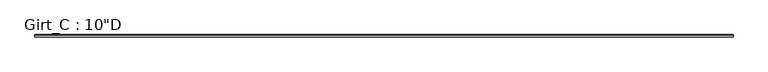
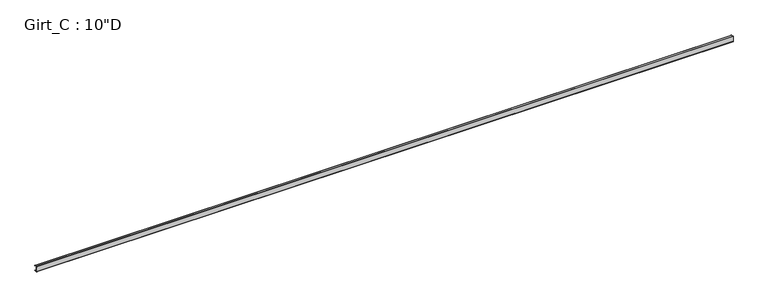
"""IFC4 building model written with IfcOpenShell, lengths in millimetres: beam geometry."""

import ifcopenshell
import ifcopenshell.guid

model = None  # the IFC model being written
_history = None  # IfcOwnerHistory: only IFC2X3 demands one
_inside = {}  # id of a spatial element -> (the spatial element, [elements in it])
_under = {}  # id of a project, library or spatial element -> (it, [spatial elements below it])
_declared = {}  # id of a project -> (the project, [libraries it declares])
_typed = {}  # id of a type object -> (the type object, [elements of that type])
_made_of = {}  # id of a material, layer set ... -> (it, [elements and type objects made of it])


def new_model(schema):
    """Start an empty IFC model of exactly this schema.

    Asked for "IFC4X3", IfcOpenShell would pick the latest addendum, in which some entities
    have other attributes; the version numbers below select the first issue.
    IFC2X3 requires an IfcOwnerHistory on every rooted entity: one is made here for all.
    """
    global model, _history
    if schema == "IFC4X3":
        model = ifcopenshell.file(schema_version=(4, 3, 0, 0))
    else:
        model = ifcopenshell.file(schema=schema)
    _inside.clear()
    _under.clear()
    _declared.clear()
    _typed.clear()
    _made_of.clear()
    _history = None
    if model.schema == "IFC2X3":
        org = make("IfcOrganization", Name="unknown")
        user = make(
            "IfcPersonAndOrganization",
            ThePerson=make("IfcPerson", FamilyName="unknown"),
            TheOrganization=org,
        )
        app = make(
            "IfcApplication",
            ApplicationDeveloper=org,
            Version="unknown",
            ApplicationFullName="unknown",
            ApplicationIdentifier="unknown",
        )
        _history = make(
            "IfcOwnerHistory",
            OwningUser=user,
            OwningApplication=app,
            ChangeAction="ADDED",
            CreationDate=0,
        )
    return model


def make(cls, **values):
    """One entity of the class cls with the attributes given. An attribute that is None is left unset."""
    return model.create_entity(
        cls, **{name: value for name, value in values.items() if value is not None}
    )


def rooted(cls, **values):
    """An entity with a GlobalId (a new one), such as an element, a storey or a relation."""
    return make(cls, GlobalId=ifcopenshell.guid.new(), OwnerHistory=_history, **values)


def si_unit(unit_type, name, prefix=None):
    """IfcSIUnit, for example si_unit("LENGTHUNIT", "METRE", prefix="MILLI")."""
    return make("IfcSIUnit", UnitType=unit_type, Prefix=prefix, Name=name)


def assignment(units):
    """IfcUnitAssignment: the units of a project."""
    return None if units is None else make("IfcUnitAssignment", Units=units)


def point(xyz):
    """IfcCartesianPoint."""
    return None if xyz is None else make("IfcCartesianPoint", Coordinates=xyz)


def direction(xyz):
    """IfcDirection."""
    return None if xyz is None else make("IfcDirection", DirectionRatios=xyz)


def frame(location, z_axis=None, x_axis=None):
    """IfcAxis2Placement3D, a coordinate frame: its origin and axes. An axis left out is left unset."""
    return make(
        "IfcAxis2Placement3D",
        Location=point(location),
        Axis=direction(z_axis),
        RefDirection=direction(x_axis),
    )


def frame_2d(location, x_axis=None):
    """IfcAxis2Placement2D, a coordinate frame in the plane: its origin and x axis."""
    return make(
        "IfcAxis2Placement2D", Location=point(location), RefDirection=direction(x_axis)
    )


def origin():
    """The frame at (0, 0, 0) with its axes left unset."""
    return frame((0.0, 0.0, 0.0))


def place(relative_to, where):
    """IfcLocalPlacement: puts the frame where relative to a parent placement (None: the world)."""
    return make(
        "IfcLocalPlacement", PlacementRelTo=relative_to, RelativePlacement=where
    )


def context(
    kind, dimensions, precision=None, world=None, true_north=None, identifier=None
):
    """IfcGeometricRepresentationContext, for example the 3D "Model" context."""
    return make(
        "IfcGeometricRepresentationContext",
        ContextIdentifier=identifier,
        ContextType=kind,
        CoordinateSpaceDimension=dimensions,
        Precision=precision,
        WorldCoordinateSystem=world,
        TrueNorth=true_north,
    )


def project(units=None, contexts=None):
    """IfcProject with its units and contexts."""
    return rooted(
        "IfcProject",
        Name="project",
        RepresentationContexts=contexts,
        UnitsInContext=assignment(units),
    )


def spatial(cls, under=None, at=None, **own):
    """A site, building, storey or space (cls), placed at a placement, below another one or the project."""
    s = rooted(cls, ObjectPlacement=at, **own)
    if under is not None:
        _under.setdefault(under.id(), (under, []))[1].append(s)
    return s


def polyline(points):
    """IfcPolyline through the points."""
    return make("IfcPolyline", Points=[point(p) for p in points])


def circle_curve(where, radius):
    """IfcCircle in the frame where."""
    return make("IfcCircle", Position=where, Radius=radius)


def trimmed(basis, trim1, trim2, sense, master):
    """IfcTrimmedCurve: the piece of a basis curve between two trims."""
    return make(
        "IfcTrimmedCurve",
        BasisCurve=basis,
        Trim1=trim1,
        Trim2=trim2,
        SenseAgreement=sense,
        MasterRepresentation=master,
    )


def segment(curve, same_sense, transition):
    """IfcCompositeCurveSegment."""
    return make(
        "IfcCompositeCurveSegment",
        Transition=transition,
        SameSense=same_sense,
        ParentCurve=curve,
    )


def composite_curve(segments, self_intersect=None):
    """IfcCompositeCurve: segments joined end to end."""
    return make("IfcCompositeCurve", Segments=segments, SelfIntersect=self_intersect)


def outline(outer, holes=None, kind="AREA"):
    """IfcArbitraryClosedProfileDef: a profile drawn as a closed curve; with holes, ...WithVoids."""
    if holes is None:
        return make("IfcArbitraryClosedProfileDef", ProfileType=kind, OuterCurve=outer)
    return make(
        "IfcArbitraryProfileDefWithVoids",
        ProfileType=kind,
        OuterCurve=outer,
        InnerCurves=holes,
    )


def extrude(swept, where, along, depth):
    """IfcExtrudedAreaSolid: the profile swept, set in the frame where, extruded along a direction by depth."""
    return make(
        "IfcExtrudedAreaSolid",
        SweptArea=swept,
        Position=where,
        ExtrudedDirection=direction(along),
        Depth=depth,
    )


def shape(context_of_items, identifier, shape_type, items):
    """IfcShapeRepresentation: the items that make up one representation, for example the "Body"."""
    return make(
        "IfcShapeRepresentation",
        ContextOfItems=context_of_items,
        RepresentationIdentifier=identifier,
        RepresentationType=shape_type,
        Items=items,
    )


def source(mapping_origin, context_of_items, identifier, shape_type, items):
    """IfcRepresentationMap: a shape defined once, which mapped items show again and again."""
    return make(
        "IfcRepresentationMap",
        MappingOrigin=mapping_origin,
        MappedRepresentation=shape(context_of_items, identifier, shape_type, items),
    )


def transform(
    local_origin,
    x_axis=None,
    y_axis=None,
    z_axis=None,
    scale=None,
    scale2=None,
    scale3=None,
    uniform=True,
):
    """IfcCartesianTransformationOperator3D, or its non-uniform kind. x_axis, y_axis, z_axis: its Axis1, 2, 3."""
    if uniform:
        return make(
            "IfcCartesianTransformationOperator3D",
            Axis1=direction(x_axis),
            Axis2=direction(y_axis),
            LocalOrigin=point(local_origin),
            Scale=scale,
            Axis3=direction(z_axis),
        )
    return make(
        "IfcCartesianTransformationOperator3DnonUniform",
        Axis1=direction(x_axis),
        Axis2=direction(y_axis),
        LocalOrigin=point(local_origin),
        Scale=scale,
        Axis3=direction(z_axis),
        Scale2=scale2,
        Scale3=scale3,
    )


def mapped(mapping_source, mapping_target):
    """IfcMappedItem: shows the shape of a source again, moved by a transform."""
    return make(
        "IfcMappedItem", MappingSource=mapping_source, MappingTarget=mapping_target
    )


def made_of(thing, what):
    """Note that an element or type object is made of a material, layer set ...; save() writes the relation."""
    if what is not None:
        _made_of.setdefault(what.id(), (what, []))[1].append(thing)
    return thing


def element(
    cls,
    number,
    at=None,
    inside=None,
    cuts=None,
    type_object=None,
    material=None,
    context=None,
    identifier="Body",
    shape_type=None,
    held_by="IfcProductDefinitionShape",
    body=None,
    shapes=None,
    **own,
):
    """One element of the class cls, such as IfcWall. Its Tag is "e" and its number.

    at: its placement. inside: the storey or other place that contains it. cuts: it is an
    opening in that element (IfcRelVoidsElement). A single representation is given by context,
    identifier, shape_type and body (its items); several are given by shapes. held_by: the class
    of the entity that holds the representations. save() writes the other relations.
    """
    e = rooted(cls, Tag="e%d" % number, ObjectPlacement=at, **own)
    if body is not None:
        shapes = [shape(context, identifier, shape_type, body)]
    if shapes is not None:
        e.Representation = make(held_by, Representations=shapes)
    if inside is not None:
        _inside.setdefault(inside.id(), (inside, []))[1].append(e)
    if cuts is not None:
        rooted(
            "IfcRelVoidsElement", RelatingBuildingElement=cuts, RelatedOpeningElement=e
        )
    if type_object is not None:
        _typed.setdefault(type_object.id(), (type_object, []))[1].append(e)
    return made_of(e, material)


def aggregate(whole, parts):
    """IfcRelAggregates: a whole, such as a stair, and the parts it consists of."""
    return rooted("IfcRelAggregates", RelatingObject=whole, RelatedObjects=parts)


def save(model, path):
    """Write the relations noted so far, then the file.

    IfcRelAggregates (storeys below a building ...), IfcRelContainedInSpatialStructure (elements
    in a storey), IfcRelDefinesByType, IfcRelAssociatesMaterial and IfcRelDeclares: one each for
    every whole, place, type object, material and project.
    """
    for whole, parts in _under.values():
        aggregate(whole, parts)
    for where, things in _inside.values():
        rooted(
            "IfcRelContainedInSpatialStructure",
            RelatedElements=things,
            RelatingStructure=where,
        )
    for kind, things in _typed.values():
        rooted("IfcRelDefinesByType", RelatedObjects=things, RelatingType=kind)
    for what, things in _made_of.values():
        rooted("IfcRelAssociatesMaterial", RelatedObjects=things, RelatingMaterial=what)
    for by, libraries in _declared.values():
        rooted("IfcRelDeclares", RelatingContext=by, RelatedDefinitions=libraries)
    model.write(path)


def beam_2726e444(model_context):
    return source(origin(), model_context, "Body", "SweptSolid", [
        extrude(outline(composite_curve([segment(polyline([(87.5109375, 127.0), (99.7560415, 112.4068534), (97.6278742, 110.621109), (86.2154765, 124.221875), (3.3005807, 124.221875)]), True, "CONTINUOUS"), segment(trimmed(circle_curve(frame_2d((3.3741066, 122.2381931)), 1.9850441), [point((3.3005807, 124.221875))], [point((1.3890625, 122.2381931))], True, "CARTESIAN"), True, "CONTINUOUS"), segment(polyline([(1.3890625, 122.2381931), (1.3890625, -122.2389339)]), True, "CONTINUOUS"), segment(trimmed(circle_curve(frame_2d((3.3748024, -122.2389339)), 1.9857399), [point((1.3890625, -122.2389339))], [point((3.2694106, -124.221875))], True, "CARTESIAN"), True, "CONTINUOUS"), segment(polyline([(3.2694106, -124.221875), (86.2154765, -124.221875), (97.6510975, -110.5934327), (99.7792647, -112.379177), (87.5109375, -127.0), (3.3734375, -127.0)]), True, "CONTINUOUS"), segment(trimmed(circle_curve(frame_2d((3.3734375, -122.2375)), 4.7625), [point((3.3734375, -127.0))], [point((-1.3890625, -122.2375))], False, "CARTESIAN"), True, "CONTINUOUS"), segment(polyline([(-1.3890625, -122.2375), (-1.3890625, 122.2375)]), True, "CONTINUOUS"), segment(trimmed(circle_curve(frame_2d((3.3734375, 122.2375)), 4.7625), [point((-1.3890625, 122.2375))], [point((3.3734375, 127.0))], False, "CARTESIAN"), True, "CONTINUOUS"), segment(polyline([(3.3734375, 127.0), (87.5109375, 127.0)]), True, "CONTINUOUS")], self_intersect=False)), frame((-15567.025, 0.0, 0.0), z_axis=(1.0, 0.0, 0.0), x_axis=(0.0, 1.0, 0.0)), (0.0, 0.0, 1.0), 31083.25),
    ])


if __name__ == "__main__":
    model = new_model("IFC4")
    model_context = context("Model", 3, world=origin())
    ifc_project = project(units=[si_unit("LENGTHUNIT", "METRE", prefix="MILLI")], contexts=[model_context])
    site = spatial("IfcSite", under=ifc_project)
    building = spatial("IfcBuilding", under=site)
    placement = place(None, origin())
    beam_shape = beam_2726e444(model_context)
    element("IfcBeam", 1, ObjectType="Girt_C : 10\"D", at=placement, inside=building, context=model_context, shape_type="MappedRepresentation", body=[
        mapped(beam_shape, transform((0.0, 0.0, 0.0), x_axis=(1.0, 0.0, 0.0), y_axis=(0.0, 1.0, 0.0), z_axis=(0.0, 0.0, 1.0))),
    ])
    save(model, "model.ifc")

# Revit data of these elements
# Type "Girt_C : 10\"D"
#   half leg = 0' - 1 3/4"
#   Web_Thickness = 0' - 0 7/64"
#   Length [instance default] = 10' - 0"
#   Leg_1 = 0' - 3 1/2"
#   Height = 0' - 10"
#   Structural Material [instance default] = none
